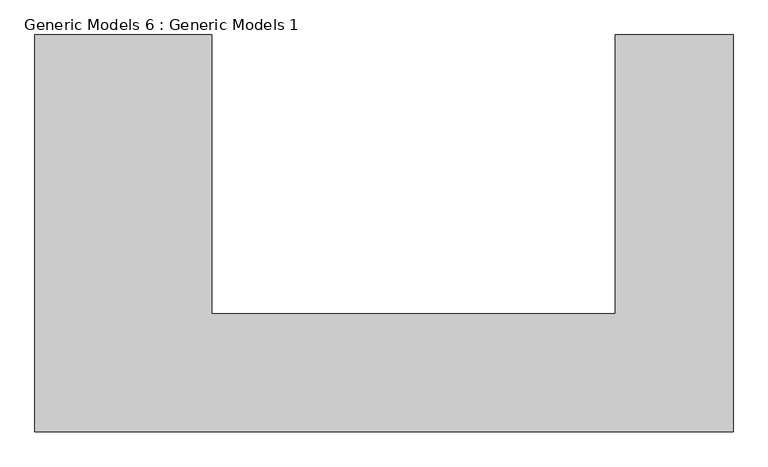
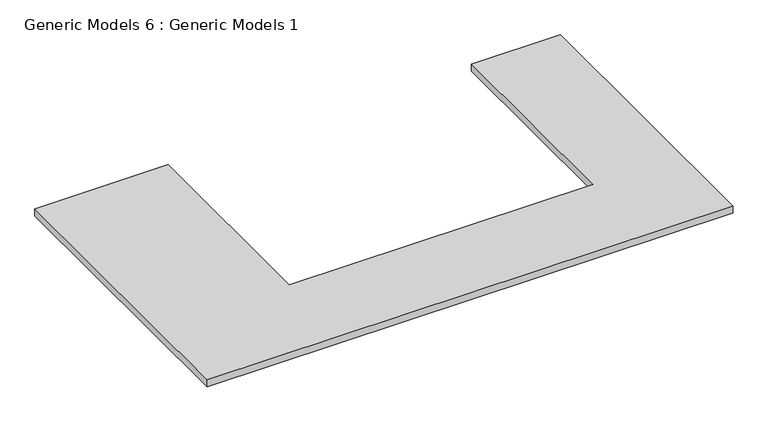
"""IFC4 building model written with IfcOpenShell, lengths in millimetres: furniture geometry, Generic Models 6 : Generic Models 1."""

from ifc_helpers import new_model, si_unit, frame, origin, place, context, project, spatial, polyline, outline, extrude, source, transform, mapped, element, save


def generic_models_6_generic_models_1_42674549(model_context):
    return source(origin(), model_context, "Body", "SweptSolid", [
        extrude(outline(polyline([(28815.9902986, -22295.2830088), (28815.9902986, -20244.2330088), (29730.3902986, -20244.2330088), (29730.3902986, -21685.6830088), (31816.3652986, -21685.6830088), (31816.3652986, -20244.2330088), (32425.9652986, -20244.2330088), (32425.9652986, -22295.2830088), (28815.9902986, -22295.2830088)])), frame((0.0, 0.0, 1016.0), z_axis=(0.0, 0.0, 1.0), x_axis=(1.0, 0.0, 0.0)), (0.0, 0.0, 1.0), 50.8),
    ])


if __name__ == "__main__":
    model = new_model("IFC4")
    model_context = context("Model", 3, world=origin())
    ifc_project = project(units=[si_unit("LENGTHUNIT", "METRE", prefix="MILLI")], contexts=[model_context])
    site = spatial("IfcSite", under=ifc_project)
    building = spatial("IfcBuilding", under=site)
    placement = place(None, origin())
    generic_models_6_generic_models_1_shape = generic_models_6_generic_models_1_42674549(model_context)
    element("IfcFurniture", 1, ObjectType="Generic Models 6 : Generic Models 1", at=placement, inside=building, context=model_context, shape_type="MappedRepresentation", body=[
        mapped(generic_models_6_generic_models_1_shape, transform((0.0, 0.0, 0.0), x_axis=(1.0, 0.0, 0.0), y_axis=(0.0, 1.0, 0.0), z_axis=(0.0, 0.0, 1.0))),
    ])
    save(model, "model.ifc")

# Revit data of these elements
# Element 1 (IfcFurniture, "Generic Models 6 : Generic Models 1")
#   Materials on its faces: "casework"
# Materials
#   "casework": class "Generic", colour RGB 209 209 209, transparency 0, Cost = 0
